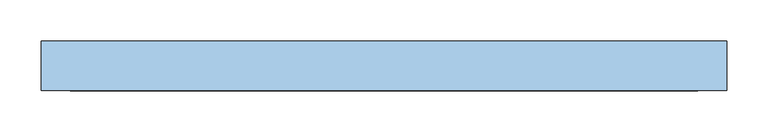
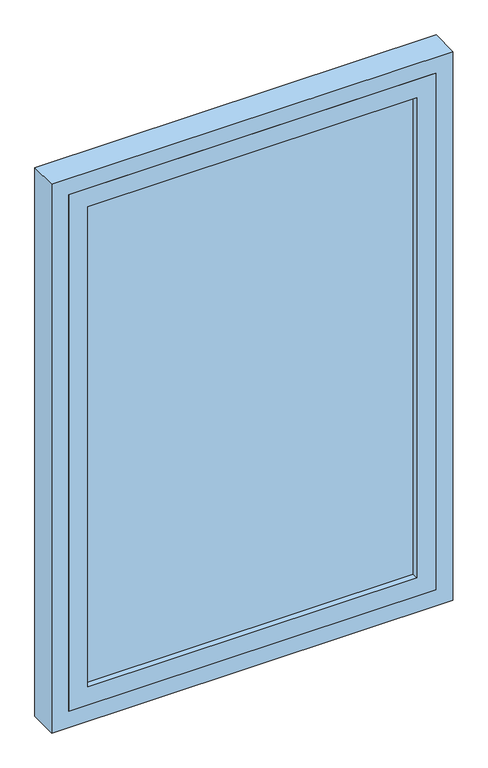
"""IFC4 building model written with IfcOpenShell, lengths in millimetres: window geometry, Janela fixa - 1 Painel : Janela fixa - 1 Painel."""

from ifc_helpers import new_model, si_unit, frame, origin, place, context, project, spatial, polyline, outline, extrude, source, transform, mapped, element, save


def window_71ad020b(model_context):
    return source(origin(), model_context, "Body", "SweptSolid", [
        extrude(outline(polyline([(340.0, -52.6), (340.0, -66.6), (-340.0, -66.6), (-340.0, -52.6), (340.0, -52.6)])), frame((0.0, 0.0, 725.0), z_axis=(0.0, 0.0, 1.0), x_axis=(1.0, 0.0, 0.0)), (0.0, 0.0, 1.0), 1050.0),
        extrude(outline(polyline([(685.0, -380.0), (685.0, 380.0), (1815.0, 380.0), (1815.0, -380.0), (685.0, -380.0)]), holes=[polyline([(1775.0, -340.0), (1775.0, 340.0), (725.0, 340.0), (725.0, -340.0), (1775.0, -340.0)])]), frame((0.0, -79.6, 0.0), z_axis=(0.0, 1.0, 0.0), x_axis=(0.0, 0.0, 1.0)), (0.0, 0.0, 1.0), 40.0),
        extrude(outline(polyline([(650.0, -415.0), (650.0, 415.0), (1850.0, 415.0), (1850.0, -415.0), (650.0, -415.0)]), holes=[polyline([(1815.0, -380.0), (1815.0, 380.0), (685.0, 380.0), (685.0, -380.0), (1815.0, -380.0)])]), frame((0.0, -79.6, 0.0), z_axis=(0.0, 1.0, 0.0), x_axis=(0.0, 0.0, 1.0)), (0.0, 0.0, 1.0), 60.0),
    ])


if __name__ == "__main__":
    model = new_model("IFC4")
    model_context = context("Model", 3, world=origin())
    ifc_project = project(units=[si_unit("LENGTHUNIT", "METRE", prefix="MILLI")], contexts=[model_context])
    site = spatial("IfcSite", under=ifc_project)
    building = spatial("IfcBuilding", under=site)
    placement = place(None, origin())
    window_shape = window_71ad020b(model_context)
    element("IfcWindow", 1, ObjectType="Janela fixa - 1 Painel : Janela fixa - 1 Painel", at=placement, inside=building, context=model_context, shape_type="MappedRepresentation", body=[
        mapped(window_shape, transform((0.0, 0.0, 0.0), x_axis=(1.0, 0.0, 0.0), y_axis=(0.0, 1.0, 0.0), z_axis=(0.0, 0.0, 1.0))),
    ])
    save(model, "model.ifc")

# Revit data of these elements
# Type "Janela fixa - 1 Painel : Janela fixa - 1 Painel"
#   Type Mark = "J15"
#   Construction Type Id = "SGL"
#   Analytic Construction = "Janelas grandes envidraçadas únicas"
#   Visual Light Transmittance = 0.9
#   Solar Heat Gain Coefficient = 0.86
#   Rough Width = 0.83 m
#   Rough Height = 1.20 m
#   Largura da moldura do painel = 0.04 m
#   Espessura da moldura do painel = 0.04 m
#   Height = 1.20 m
#   Heat Transfer Coefficient (U) = 5.5617 W/(m²·K)
#   Largura da estrutura = 0.035 m
#   Espessura da moldura = 0.06 m
#   Altura-padrão do peitoril = 0.65 m
#   Width = 0.83 m
#   Vidro = Vidro - Janela
#   Material da estrutura = Aluminum Sill
#   Wall Closure = (empty or 0)
# Element 1 (IfcWindow, "Janela fixa - 1 Painel : Janela fixa - 1 Painel")
#   Materials on its faces: "Aluminum Sill", "Vidro - Janela"
# Materials
#   "Vidro - Janela": class "Vidro", colour RGB 249 249 249, transparency 1, Cost = 0
#   "Aluminum Sill": class "Não atribuído", colour RGB 247 247 247, transparency 0
